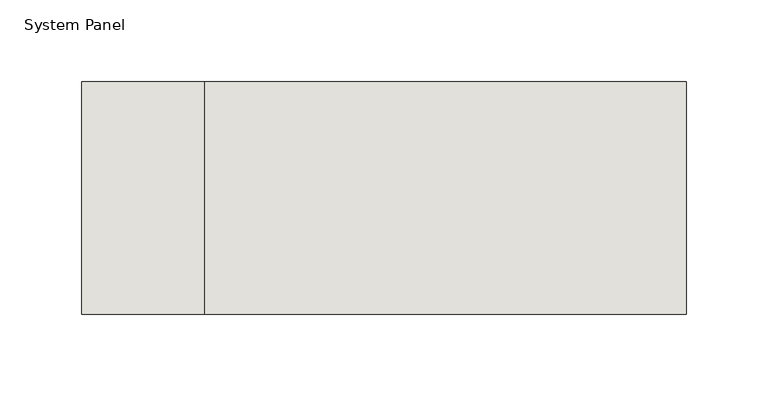
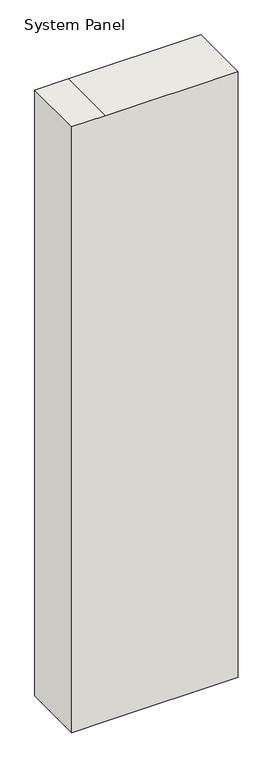
"""IFC4 building model written with IfcOpenShell, lengths in millimetres: wall geometry, System Panel : NLRS_21_CWP_hsb-vulling minerale wol 142 _gen_rsf."""

from ifc_helpers import new_model, si_unit, frame, origin, place, context, project, spatial, polyline, outline, extrude, source, transform, mapped, element, save


def system_panel_a8f59ee8(model_context):
    return source(origin(), model_context, "Body", "SweptSolid", [
        extrude(outline(polyline([(0.0, -184.5), (0.0, -109.3441061), (0.0, 184.5), (1421.0, 184.5), (1421.0, -109.3441061), (1421.0, -184.5), (0.0, -184.5)])), frame((0.0, -71.0, 0.0), z_axis=(0.0, 1.0, 0.0), x_axis=(0.0, 0.0, 1.0)), (0.0, 0.0, 1.0), 142.0),
    ])


if __name__ == "__main__":
    model = new_model("IFC4")
    model_context = context("Model", 3, world=origin())
    ifc_project = project(units=[si_unit("LENGTHUNIT", "METRE", prefix="MILLI")], contexts=[model_context])
    site = spatial("IfcSite", under=ifc_project)
    building = spatial("IfcBuilding", under=site)
    placement = place(None, origin())
    system_panel_shape = system_panel_a8f59ee8(model_context)
    element("IfcWall", 1, ObjectType="System Panel : NLRS_21_CWP_hsb-vulling minerale wol 142 _gen_rsf", at=placement, inside=building, context=model_context, shape_type="MappedRepresentation", body=[
        mapped(system_panel_shape, transform((0.0, 0.0, 0.0), x_axis=(1.0, 0.0, 0.0), y_axis=(0.0, 1.0, 0.0), z_axis=(0.0, 0.0, 1.0))),
    ])
    save(model, "model.ifc")

# Revit data of these elements
# Type "System Panel : NLRS_21_CWP_hsb-vulling minerale wol 142 _gen_rsf"
#   Type IfcGUID = "07M7mRoiH1CR8m_RSKIwpC"
#   Assembly Code = "21.23"
#   IfcExportAs = "IfcWall"
# Element 1 (IfcWall, "System Panel : NLRS_21_CWP_hsb-vulling minerale wol 142 _gen_rsf")
#   Materials on its faces: "NLRS_m1_isolatie minerale wol_gen_rsf"
# Materials
#   "NLRS_m1_isolatie minerale wol_gen_rsf": class "M - Anorganische materialen", colour RGB 200 200 140, transparency 0, Keynote = "m1", Manufacturer = "Revit Standards Foundation", URL = "www.revitstandards.org", Description = "isolatie minerale wol", Cost = 0
